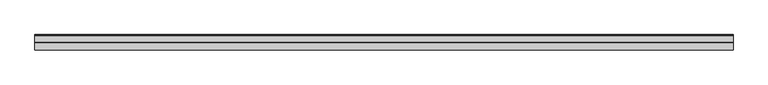
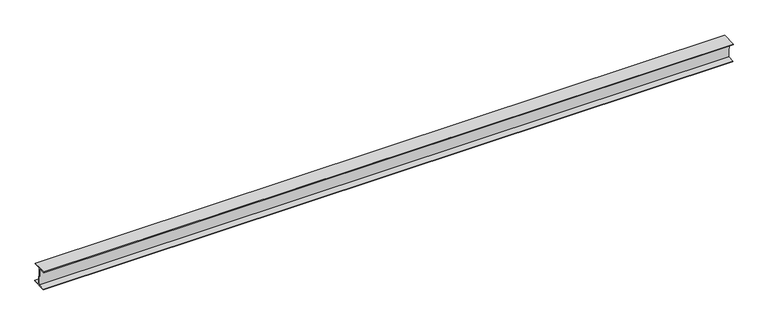
"""IFC4 building model written with IfcOpenShell, lengths in millimetres: proxy geometry, Generic Models 7:Generic Models 1:8:Generic Models 1:8 : Generic Models 7:Generic Models 1:337419:49 : Generic Models 7:Generic Models 1:8:Generic Models 1:8 : Generic Models 7:Generic Models 1:337419:315935."""

import ifcopenshell
import ifcopenshell.guid

model = None  # the IFC model being written
_history = None  # IfcOwnerHistory: only IFC2X3 demands one
_inside = {}  # id of a spatial element -> (the spatial element, [elements in it])
_under = {}  # id of a project, library or spatial element -> (it, [spatial elements below it])
_declared = {}  # id of a project -> (the project, [libraries it declares])
_typed = {}  # id of a type object -> (the type object, [elements of that type])
_made_of = {}  # id of a material, layer set ... -> (it, [elements and type objects made of it])


def new_model(schema):
    """Start an empty IFC model of exactly this schema.

    Asked for "IFC4X3", IfcOpenShell would pick the latest addendum, in which some entities
    have other attributes; the version numbers below select the first issue.
    IFC2X3 requires an IfcOwnerHistory on every rooted entity: one is made here for all.
    """
    global model, _history
    if schema == "IFC4X3":
        model = ifcopenshell.file(schema_version=(4, 3, 0, 0))
    else:
        model = ifcopenshell.file(schema=schema)
    _inside.clear()
    _under.clear()
    _declared.clear()
    _typed.clear()
    _made_of.clear()
    _history = None
    if model.schema == "IFC2X3":
        org = make("IfcOrganization", Name="unknown")
        user = make(
            "IfcPersonAndOrganization",
            ThePerson=make("IfcPerson", FamilyName="unknown"),
            TheOrganization=org,
        )
        app = make(
            "IfcApplication",
            ApplicationDeveloper=org,
            Version="unknown",
            ApplicationFullName="unknown",
            ApplicationIdentifier="unknown",
        )
        _history = make(
            "IfcOwnerHistory",
            OwningUser=user,
            OwningApplication=app,
            ChangeAction="ADDED",
            CreationDate=0,
        )
    return model


def make(cls, **values):
    """One entity of the class cls with the attributes given. An attribute that is None is left unset."""
    return model.create_entity(
        cls, **{name: value for name, value in values.items() if value is not None}
    )


def rooted(cls, **values):
    """An entity with a GlobalId (a new one), such as an element, a storey or a relation."""
    return make(cls, GlobalId=ifcopenshell.guid.new(), OwnerHistory=_history, **values)


def si_unit(unit_type, name, prefix=None):
    """IfcSIUnit, for example si_unit("LENGTHUNIT", "METRE", prefix="MILLI")."""
    return make("IfcSIUnit", UnitType=unit_type, Prefix=prefix, Name=name)


def assignment(units):
    """IfcUnitAssignment: the units of a project."""
    return None if units is None else make("IfcUnitAssignment", Units=units)


def point(xyz):
    """IfcCartesianPoint."""
    return None if xyz is None else make("IfcCartesianPoint", Coordinates=xyz)


def direction(xyz):
    """IfcDirection."""
    return None if xyz is None else make("IfcDirection", DirectionRatios=xyz)


def frame(location, z_axis=None, x_axis=None):
    """IfcAxis2Placement3D, a coordinate frame: its origin and axes. An axis left out is left unset."""
    return make(
        "IfcAxis2Placement3D",
        Location=point(location),
        Axis=direction(z_axis),
        RefDirection=direction(x_axis),
    )


def origin():
    """The frame at (0, 0, 0) with its axes left unset."""
    return frame((0.0, 0.0, 0.0))


def place(relative_to, where):
    """IfcLocalPlacement: puts the frame where relative to a parent placement (None: the world)."""
    return make(
        "IfcLocalPlacement", PlacementRelTo=relative_to, RelativePlacement=where
    )


def context(
    kind, dimensions, precision=None, world=None, true_north=None, identifier=None
):
    """IfcGeometricRepresentationContext, for example the 3D "Model" context."""
    return make(
        "IfcGeometricRepresentationContext",
        ContextIdentifier=identifier,
        ContextType=kind,
        CoordinateSpaceDimension=dimensions,
        Precision=precision,
        WorldCoordinateSystem=world,
        TrueNorth=true_north,
    )


def project(units=None, contexts=None):
    """IfcProject with its units and contexts."""
    return rooted(
        "IfcProject",
        Name="project",
        RepresentationContexts=contexts,
        UnitsInContext=assignment(units),
    )


def spatial(cls, under=None, at=None, **own):
    """A site, building, storey or space (cls), placed at a placement, below another one or the project."""
    s = rooted(cls, ObjectPlacement=at, **own)
    if under is not None:
        _under.setdefault(under.id(), (under, []))[1].append(s)
    return s


def polyline(points):
    """IfcPolyline through the points."""
    return make("IfcPolyline", Points=[point(p) for p in points])


def outline(outer, holes=None, kind="AREA"):
    """IfcArbitraryClosedProfileDef: a profile drawn as a closed curve; with holes, ...WithVoids."""
    if holes is None:
        return make("IfcArbitraryClosedProfileDef", ProfileType=kind, OuterCurve=outer)
    return make(
        "IfcArbitraryProfileDefWithVoids",
        ProfileType=kind,
        OuterCurve=outer,
        InnerCurves=holes,
    )


def extrude(swept, where, along, depth):
    """IfcExtrudedAreaSolid: the profile swept, set in the frame where, extruded along a direction by depth."""
    return make(
        "IfcExtrudedAreaSolid",
        SweptArea=swept,
        Position=where,
        ExtrudedDirection=direction(along),
        Depth=depth,
    )


def shape(context_of_items, identifier, shape_type, items):
    """IfcShapeRepresentation: the items that make up one representation, for example the "Body"."""
    return make(
        "IfcShapeRepresentation",
        ContextOfItems=context_of_items,
        RepresentationIdentifier=identifier,
        RepresentationType=shape_type,
        Items=items,
    )


def source(mapping_origin, context_of_items, identifier, shape_type, items):
    """IfcRepresentationMap: a shape defined once, which mapped items show again and again."""
    return make(
        "IfcRepresentationMap",
        MappingOrigin=mapping_origin,
        MappedRepresentation=shape(context_of_items, identifier, shape_type, items),
    )


def transform(
    local_origin,
    x_axis=None,
    y_axis=None,
    z_axis=None,
    scale=None,
    scale2=None,
    scale3=None,
    uniform=True,
):
    """IfcCartesianTransformationOperator3D, or its non-uniform kind. x_axis, y_axis, z_axis: its Axis1, 2, 3."""
    if uniform:
        return make(
            "IfcCartesianTransformationOperator3D",
            Axis1=direction(x_axis),
            Axis2=direction(y_axis),
            LocalOrigin=point(local_origin),
            Scale=scale,
            Axis3=direction(z_axis),
        )
    return make(
        "IfcCartesianTransformationOperator3DnonUniform",
        Axis1=direction(x_axis),
        Axis2=direction(y_axis),
        LocalOrigin=point(local_origin),
        Scale=scale,
        Axis3=direction(z_axis),
        Scale2=scale2,
        Scale3=scale3,
    )


def mapped(mapping_source, mapping_target):
    """IfcMappedItem: shows the shape of a source again, moved by a transform."""
    return make(
        "IfcMappedItem", MappingSource=mapping_source, MappingTarget=mapping_target
    )


def made_of(thing, what):
    """Note that an element or type object is made of a material, layer set ...; save() writes the relation."""
    if what is not None:
        _made_of.setdefault(what.id(), (what, []))[1].append(thing)
    return thing


def element(
    cls,
    number,
    at=None,
    inside=None,
    cuts=None,
    type_object=None,
    material=None,
    context=None,
    identifier="Body",
    shape_type=None,
    held_by="IfcProductDefinitionShape",
    body=None,
    shapes=None,
    **own,
):
    """One element of the class cls, such as IfcWall. Its Tag is "e" and its number.

    at: its placement. inside: the storey or other place that contains it. cuts: it is an
    opening in that element (IfcRelVoidsElement). A single representation is given by context,
    identifier, shape_type and body (its items); several are given by shapes. held_by: the class
    of the entity that holds the representations. save() writes the other relations.
    """
    e = rooted(cls, Tag="e%d" % number, ObjectPlacement=at, **own)
    if body is not None:
        shapes = [shape(context, identifier, shape_type, body)]
    if shapes is not None:
        e.Representation = make(held_by, Representations=shapes)
    if inside is not None:
        _inside.setdefault(inside.id(), (inside, []))[1].append(e)
    if cuts is not None:
        rooted(
            "IfcRelVoidsElement", RelatingBuildingElement=cuts, RelatedOpeningElement=e
        )
    if type_object is not None:
        _typed.setdefault(type_object.id(), (type_object, []))[1].append(e)
    return made_of(e, material)


def aggregate(whole, parts):
    """IfcRelAggregates: a whole, such as a stair, and the parts it consists of."""
    return rooted("IfcRelAggregates", RelatingObject=whole, RelatedObjects=parts)


def save(model, path):
    """Write the relations noted so far, then the file.

    IfcRelAggregates (storeys below a building ...), IfcRelContainedInSpatialStructure (elements
    in a storey), IfcRelDefinesByType, IfcRelAssociatesMaterial and IfcRelDeclares: one each for
    every whole, place, type object, material and project.
    """
    for whole, parts in _under.values():
        aggregate(whole, parts)
    for where, things in _inside.values():
        rooted(
            "IfcRelContainedInSpatialStructure",
            RelatedElements=things,
            RelatingStructure=where,
        )
    for kind, things in _typed.values():
        rooted("IfcRelDefinesByType", RelatedObjects=things, RelatingType=kind)
    for what, things in _made_of.values():
        rooted("IfcRelAssociatesMaterial", RelatedObjects=things, RelatingMaterial=what)
    for by, libraries in _declared.values():
        rooted("IfcRelDeclares", RelatingContext=by, RelatedDefinitions=libraries)
    model.write(path)


def generic_models_ecd19c88(model_context):
    return source(origin(), model_context, "Body", "SweptSolid", [
        extrude(outline(polyline([(-576429.5235686, 4024.8210459), (-576429.7959773, 4031.6736335), (-576277.5162517, 4037.7271598), (-576277.243843, 4030.8745722), (-576350.4650111, 4027.963835), (-576342.93846, 3838.6293762), (-576269.7357554, 3841.5393794), (-576269.4633467, 3834.6867918), (-576421.7430723, 3828.6332655), (-576422.015481, 3835.4858531), (-576349.0296491, 3838.3872351), (-576356.5562001, 4027.7216939), (-576429.5235686, 4024.8210459)])), frame((608476.4367239, 0.0, 0.0), z_axis=(1.0, 0.0, 0.0), x_axis=(0.0, 1.0, 0.0)), (0.0, 0.0, 1.0), 7315.2),
    ])


if __name__ == "__main__":
    model = new_model("IFC4")
    model_context = context("Model", 3, world=origin())
    ifc_project = project(units=[si_unit("LENGTHUNIT", "METRE", prefix="MILLI")], contexts=[model_context])
    site = spatial("IfcSite", under=ifc_project)
    building = spatial("IfcBuilding", under=site)
    placement = place(None, origin())
    generic_models_shape = generic_models_ecd19c88(model_context)
    element("IfcBuildingElementProxy", 1, Name="Generic Models 7:Generic Models 1:8:Generic Models 1:8 : Generic Models 7:Generic Models 1:337419:49 : Generic Models 7:Generic Models 1:8:Generic Models 1:8 : Generic Models 7:Generic Models 1:337419:315935", ObjectType="Generic Models 7:Generic Models 1:8:Generic Models 1:8 : Generic Models 7:Generic Models 1:337419:49 : Generic Models 7:Generic Models 1:8:Generic Models 1:8 : Generic Models 7:Generic Models 1:337419:315935", at=placement, inside=building, context=model_context, shape_type="MappedRepresentation", body=[
        mapped(generic_models_shape, transform((0.0, 0.0, 0.0), x_axis=(1.0, 0.0, 0.0), y_axis=(0.0, 1.0, 0.0), z_axis=(0.0, 0.0, 1.0))),
    ])
    save(model, "model.ifc")

# Revit data of these elements
# Type "Generic Models 7:Generic Models 1:8:Generic Models 1:8 : Generic Models 7:Generic Models 1:337419:49 : Generic Models 7:Generic Models 1:8:Generic Models 1:8 : Generic Models 7:Generic Models 1:337419:315935"
#   NameOverride = "Generic Models 7:Generic Models 1:8:Generic Models 1:8 : Generic Models 7:Generic Models 1:337419:315935"
#   ObjectTypeOverride = "Generic Models 1:8 : Generic Models 7:Generic Models 1:337419"
#   Reference = "Generic Models 1"
#   Tag = "315935"
# Element 1 (IfcBuildingElementProxy, "Generic Models 7:Generic Models 1:8:Generic Models 1:8 : Generic Models 7:Generic Models 1:337419:49 : Generic Models 7:Generic Models 1:8:Generic Models 1:8 : Generic Models 7:Generic Models 1:337419:315935")
#   Materials on its faces: "STRUCTURAL STEEL - SEE STRUCT. DWGS"
# Materials
#   "STRUCTURAL STEEL - SEE STRUCT. DWGS": class "Metal", colour RGB 189 187 185, transparency 0, Description = "Structural steel 50ksi", Cost = 0
